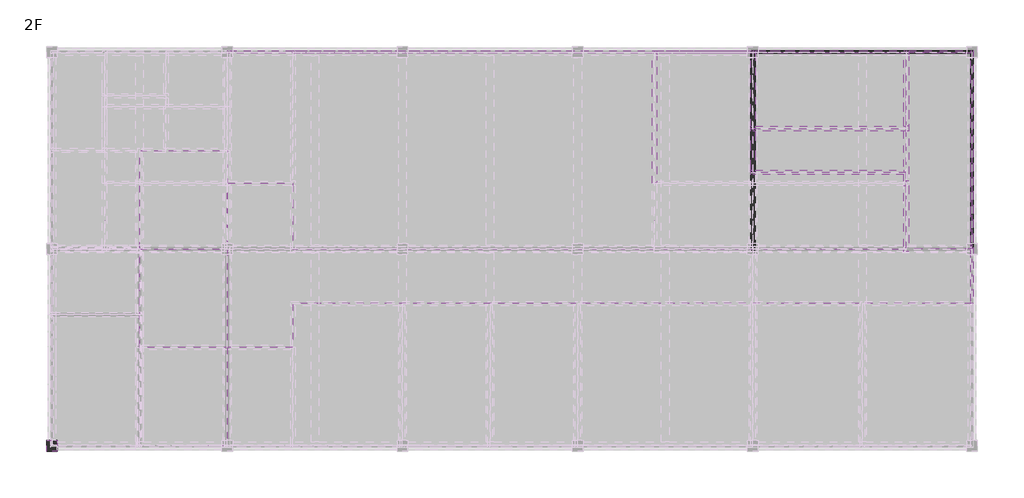
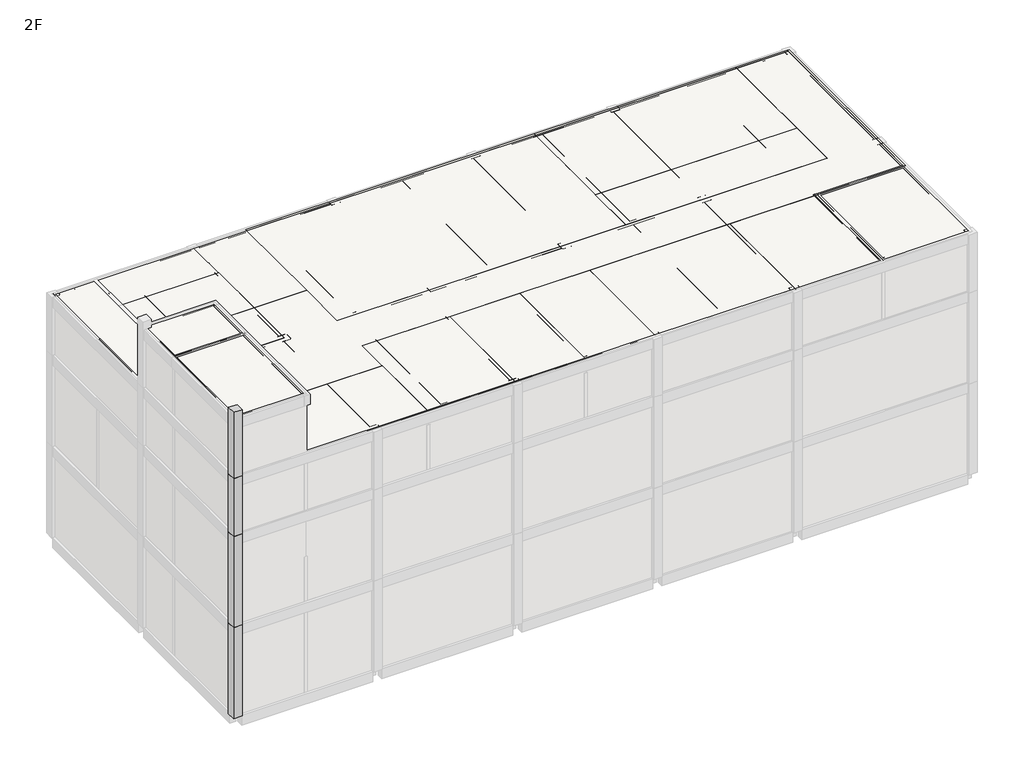
# One storey, part 3 of 7: 58 slabs, 19 walls, 4 columns.
"""IFC4 building model written with IfcOpenShell, lengths in millimetres."""

from ifc_helpers import new_model, si_unit, frame, origin, place, context, project, spatial, polyline, outline, extrude, faceted_brep, element, save

model = new_model("IFC4")

# Units and contexts
model_context = context("Model", 3, world=origin())
ifc_project = project(units=[si_unit("LENGTHUNIT", "METRE", prefix="MILLI")], contexts=[model_context])

# Site, building, storey
site = spatial("IfcSite", under=ifc_project)
building = spatial("IfcBuilding", under=site)
storey = spatial("IfcBuildingStorey", under=building, Name="2F", Elevation=3500.0)

# Columns
placement = place(None, origin())
element("IfcColumn", 1, ObjectType="Concrete-Rectangular-Column : CL111_500x500", at=placement, inside=storey, context=model_context, shape_type="Brep", body=[
    faceted_brep([(45709.6521483, 164173.8614395, 3500.0), (45709.6521483, 163673.8614395, 3500.0), (45209.6521483, 163673.8614395, 3500.0), (45209.6521483, 164173.8614395, 3500.0), (45709.6521483, 164173.8614395, 9000.0), (45709.6521483, 164098.8614395, 9000.0), (45709.6521483, 163748.8614395, 9000.0), (45709.6521483, 163673.8614395, 9000.0), (45209.6521483, 163673.8614395, 9000.0), (45209.6521483, 164173.8614395, 9000.0), (45284.6521483, 164173.8614395, 9000.0), (45634.6521483, 164173.8614395, 9000.0)], [[[0, 1, 2, 3]], [[4, 5, 6, 7, 1, 0]], [[7, 8, 2, 1]], [[8, 9, 3, 2]], [[9, 10, 11, 4, 0, 3]], [[4, 11, 10, 9, 8, 7, 6, 5]]]),
])
element("IfcColumn", 2, ObjectType="Concrete-Rectangular-Column : CL111_500x500", at=placement, inside=storey, context=model_context, shape_type="Brep", body=[
    faceted_brep([(45709.6521483, 164173.8614395, 9000.0), (45709.6521483, 163673.8614395, 9000.0), (45209.6521483, 163673.8614395, 9000.0), (45209.6521483, 164173.8614395, 9000.0), (45709.6521483, 164173.8614395, 14500.0), (45709.6521483, 164098.8614395, 14500.0), (45709.6521483, 163748.8614395, 14500.0), (45709.6521483, 163673.8614395, 14500.0), (45209.6521483, 163673.8614395, 14500.0), (45209.6521483, 164173.8614395, 14500.0), (45284.6521483, 164173.8614395, 14500.0), (45634.6521483, 164173.8614395, 14500.0)], [[[0, 1, 2, 3]], [[4, 5, 6, 7, 1, 0]], [[7, 8, 2, 1]], [[8, 9, 3, 2]], [[9, 10, 11, 4, 0, 3]], [[4, 11, 10, 9, 8, 7, 6, 5]]]),
])
element("IfcColumn", 3, ObjectType="Concrete-Rectangular-Column : CL111_500x500", at=placement, inside=storey, context=model_context, shape_type="Brep", body=[
    faceted_brep([(45709.6521483, 164173.8614395, 14500.0), (45709.6521483, 163673.8614395, 14500.0), (45209.6521483, 163673.8614395, 14500.0), (45209.6521483, 164173.8614395, 14500.0), (45709.6521483, 164173.8614395, 18000.0), (45709.6521483, 164098.8614395, 18000.0), (45709.6521483, 163748.8614395, 18000.0), (45709.6521483, 163673.8614395, 18000.0), (45209.6521483, 163673.8614395, 18000.0), (45209.6521483, 164173.8614395, 18000.0), (45284.6521483, 164173.8614395, 18000.0), (45634.6521483, 164173.8614395, 18000.0)], [[[0, 1, 2, 3]], [[4, 5, 6, 7, 1, 0]], [[7, 8, 2, 1]], [[8, 9, 3, 2]], [[9, 10, 11, 4, 0, 3]], [[4, 11, 10, 9, 8, 7, 6, 5]]]),
])
element("IfcColumn", 4, ObjectType="Concrete-Rectangular-Column : CL111_500x500", at=placement, inside=storey, context=model_context, shape_type="SweptSolid", body=[
    extrude(outline(polyline([(45709.6521483, 164173.8614395), (45709.6521483, 163673.8614395), (45209.6521483, 163673.8614395), (45209.6521483, 164173.8614395), (45709.6521483, 164173.8614395)])), frame((0.0, 0.0, 18000.0), z_axis=(0.0, 0.0, 1.0), x_axis=(1.0, 0.0, 0.0)), (0.0, 0.0, 1.0), 4000.0),
])

# Slabs
element("IfcSlab", 5, ObjectType="CFS11_Slab RC_T150", at=placement, inside=storey, context=model_context, shape_type="SweptSolid", body=[
    extrude(outline(polyline([(77459.6521483, 181923.8614395), (77459.6521483, 172923.8614395), (45459.6521483, 172923.8614395), (45459.6521483, 181923.8614395), (77459.6521483, 181923.8614395)])), frame((0.0, 0.0, 3350.0), z_axis=(0.0, 0.0, 1.0), x_axis=(1.0, 0.0, 0.0)), (0.0, 0.0, 1.0), 150.0),
])
element("IfcSlab", 6, ObjectType="CFS11_Slab RC_T150", at=placement, inside=storey, context=model_context, shape_type="SweptSolid", body=[
    extrude(outline(polyline([(53459.6521483, 163923.8614395), (53459.6521483, 172923.8614395), (87459.6521483, 172923.8614395), (87459.6521483, 163923.8614395), (53459.6521483, 163923.8614395)])), frame((0.0, 0.0, 3350.0), z_axis=(0.0, 0.0, 1.0), x_axis=(1.0, 0.0, 0.0)), (0.0, 0.0, 1.0), 150.0),
])
element("IfcSlab", 7, ObjectType="CFS11_Slab RC_T150", at=placement, inside=storey, context=model_context, shape_type="SweptSolid", body=[
    extrude(outline(polyline([(77459.6521483, 181923.8614395), (87459.6521483, 181923.8614395), (87459.6521483, 172923.8614395), (77459.6521483, 172923.8614395), (77459.6521483, 181923.8614395)])), frame((0.0, 0.0, 3350.0), z_axis=(0.0, 0.0, 1.0), x_axis=(1.0, 0.0, 0.0)), (0.0, 0.0, 1.0), 150.0),
])
element("IfcSlab", 8, ObjectType="CFS11_Slab RC_T150", at=placement, inside=storey, context=model_context, shape_type="SweptSolid", body=[
    extrude(outline(polyline([(53459.6521483, 172923.8614395), (53459.6521483, 163923.8614395), (49459.6521483, 163923.8614395), (49459.6521483, 172923.8614395), (53459.6521483, 172923.8614395)])), frame((0.0, 0.0, 3350.0), z_axis=(0.0, 0.0, 1.0), x_axis=(1.0, 0.0, 0.0)), (0.0, 0.0, 1.0), 150.0),
])
element("IfcSlab", 9, ObjectType="CFS11_Slab RC_T150", at=placement, inside=storey, context=model_context, shape_type="SweptSolid", body=[
    extrude(outline(polyline([(49459.6521483, 172923.8614395), (49459.6521483, 169923.8614395), (45459.6521483, 169923.8614395), (45459.6521483, 172923.8614395), (49459.6521483, 172923.8614395)])), frame((0.0, 0.0, 3350.0), z_axis=(0.0, 0.0, 1.0), x_axis=(1.0, 0.0, 0.0)), (0.0, 0.0, 1.0), 150.0),
])
element("IfcSlab", 10, ObjectType="CFS11_Slab RC_T150", at=placement, inside=storey, context=model_context, shape_type="SweptSolid", body=[
    extrude(outline(polyline([(49459.6521483, 163923.8614395), (45459.6521483, 163923.8614395), (45459.6521483, 169923.8614395), (49459.6521483, 169923.8614395), (49459.6521483, 163923.8614395)])), frame((0.0, 0.0, 3350.0), z_axis=(0.0, 0.0, 1.0), x_axis=(1.0, 0.0, 0.0)), (0.0, 0.0, 1.0), 150.0),
])
element("IfcSlab", 11, ObjectType="CFS11_Slab RC_T150", at=placement, inside=storey, context=model_context, shape_type="SweptSolid", body=[
    extrude(outline(polyline([(53459.6521483, 181923.8614395), (77459.6521483, 181923.8614395), (77459.6521483, 172923.8614395), (53459.6521483, 172923.8614395), (53459.6521483, 181923.8614395)])), frame((0.0, 0.0, 8850.0), z_axis=(0.0, 0.0, 1.0), x_axis=(1.0, 0.0, 0.0)), (0.0, 0.0, 1.0), 150.0),
])
element("IfcSlab", 12, ObjectType="CFS11_Slab RC_T150", at=placement, inside=storey, context=model_context, shape_type="SweptSolid", body=[
    extrude(outline(polyline([(77459.6521483, 172923.8614395), (77459.6521483, 163923.8614395), (53459.6521483, 163923.8614395), (53459.6521483, 172923.8614395), (77459.6521483, 172923.8614395)])), frame((0.0, 0.0, 8850.0), z_axis=(0.0, 0.0, 1.0), x_axis=(1.0, 0.0, 0.0)), (0.0, 0.0, 1.0), 150.0),
])
element("IfcSlab", 13, ObjectType="CFS11_Slab RC_T150", at=placement, inside=storey, context=model_context, shape_type="SweptSolid", body=[
    extrude(outline(polyline([(77459.6521483, 181923.8614395), (84459.6521483, 181923.8614395), (84459.6521483, 178423.8614395), (77459.6521483, 178423.8614395), (77459.6521483, 181923.8614395)])), frame((0.0, 0.0, 8850.0), z_axis=(0.0, 0.0, 1.0), x_axis=(1.0, 0.0, 0.0)), (0.0, 0.0, 1.0), 150.0),
])
element("IfcSlab", 14, ObjectType="CFS11_Slab RC_T150", at=placement, inside=storey, context=model_context, shape_type="SweptSolid", body=[
    extrude(outline(polyline([(77459.6521483, 163923.8614395), (77459.6521483, 172923.8614395), (87459.6521483, 172923.8614395), (87459.6521483, 163923.8614395), (77459.6521483, 163923.8614395)])), frame((0.0, 0.0, 8850.0), z_axis=(0.0, 0.0, 1.0), x_axis=(1.0, 0.0, 0.0)), (0.0, 0.0, 1.0), 150.0),
])
element("IfcSlab", 15, ObjectType="CFS11_Slab RC_T150", at=placement, inside=storey, context=model_context, shape_type="SweptSolid", body=[
    extrude(outline(polyline([(77459.6521483, 176423.8614395), (84459.6521483, 176423.8614395), (84459.6521483, 172923.8614395), (77459.6521483, 172923.8614395), (77459.6521483, 176423.8614395)])), frame((0.0, 0.0, 8850.0), z_axis=(0.0, 0.0, 1.0), x_axis=(1.0, 0.0, 0.0)), (0.0, 0.0, 1.0), 150.0),
])
element("IfcSlab", 16, ObjectType="CFS11_Slab RC_T150", at=placement, inside=storey, context=model_context, shape_type="SweptSolid", body=[
    extrude(outline(polyline([(45459.6521483, 181923.8614395), (47859.6521483, 181923.8614395), (47859.6521483, 177423.8614395), (45459.6521483, 177423.8614395), (45459.6521483, 181923.8614395)])), frame((0.0, 0.0, 8850.0), z_axis=(0.0, 0.0, 1.0), x_axis=(1.0, 0.0, 0.0)), (0.0, 0.0, 1.0), 150.0),
])
element("IfcSlab", 17, ObjectType="CFS11_Slab RC_T150", at=placement, inside=storey, context=model_context, shape_type="SweptSolid", body=[
    extrude(outline(polyline([(45459.6521483, 172923.8614395), (45459.6521483, 177423.8614395), (49459.6521483, 177423.8614395), (49459.6521483, 172923.8614395), (45459.6521483, 172923.8614395)])), frame((0.0, 0.0, 8850.0), z_axis=(0.0, 0.0, 1.0), x_axis=(1.0, 0.0, 0.0)), (0.0, 0.0, 1.0), 150.0),
])
element("IfcSlab", 18, ObjectType="CFS11_Slab RC_T150", at=placement, inside=storey, context=model_context, shape_type="SweptSolid", body=[
    extrude(outline(polyline([(53459.6521483, 177423.8614395), (50659.6521483, 177423.8614395), (50659.6521483, 181923.8614395), (53459.6521483, 181923.8614395), (53459.6521483, 177423.8614395)])), frame((0.0, 0.0, 8850.0), z_axis=(0.0, 0.0, 1.0), x_axis=(1.0, 0.0, 0.0)), (0.0, 0.0, 1.0), 150.0),
])
element("IfcSlab", 19, ObjectType="CFS11_Slab RC_T150", at=placement, inside=storey, context=model_context, shape_type="SweptSolid", body=[
    extrude(outline(polyline([(47859.6521483, 181923.8614395), (50659.6521483, 181923.8614395), (50659.6521483, 179923.8614395), (47859.6521483, 179923.8614395), (47859.6521483, 181923.8614395)])), frame((0.0, 0.0, 8850.0), z_axis=(0.0, 0.0, 1.0), x_axis=(1.0, 0.0, 0.0)), (0.0, 0.0, 1.0), 150.0),
])
element("IfcSlab", 20, ObjectType="CFS11_Slab RC_T150", at=placement, inside=storey, context=model_context, shape_type="SweptSolid", body=[
    extrude(outline(polyline([(47859.6521483, 179923.8614395), (50659.6521483, 179923.8614395), (50659.6521483, 177423.8614395), (47859.6521483, 177423.8614395), (47859.6521483, 179923.8614395)])), frame((0.0, 0.0, 8850.0), z_axis=(0.0, 0.0, 1.0), x_axis=(1.0, 0.0, 0.0)), (0.0, 0.0, 1.0), 150.0),
])
element("IfcSlab", 21, ObjectType="CFS11_Slab RC_T150", at=placement, inside=storey, context=model_context, shape_type="SweptSolid", body=[
    extrude(outline(polyline([(49459.6521483, 172923.8614395), (49459.6521483, 169923.8614395), (45459.6521483, 169923.8614395), (45459.6521483, 172923.8614395), (49459.6521483, 172923.8614395)])), frame((0.0, 0.0, 8850.0), z_axis=(0.0, 0.0, 1.0), x_axis=(1.0, 0.0, 0.0)), (0.0, 0.0, 1.0), 150.0),
])
element("IfcSlab", 22, ObjectType="CFS11_Slab RC_T150", at=placement, inside=storey, context=model_context, shape_type="SweptSolid", body=[
    extrude(outline(polyline([(49459.6521483, 169923.8614395), (49459.6521483, 163923.8614395), (45459.6521483, 163923.8614395), (45459.6521483, 169923.8614395), (49459.6521483, 169923.8614395)])), frame((0.0, 0.0, 8850.0), z_axis=(0.0, 0.0, 1.0), x_axis=(1.0, 0.0, 0.0)), (0.0, 0.0, 1.0), 150.0),
])
element("IfcSlab", 23, ObjectType="CFS11_Slab RC_T150", at=placement, inside=storey, context=model_context, shape_type="SweptSolid", body=[
    extrude(outline(polyline([(77459.6521483, 178423.8614395), (84459.6521483, 178423.8614395), (84459.6521483, 181923.8614395), (87459.6521483, 181923.8614395), (87459.6521483, 172923.8614395), (84459.6521483, 172923.8614395), (84459.6521483, 176423.8614395), (77459.6521483, 176423.8614395), (77459.6521483, 178423.8614395)])), frame((0.0, 0.0, 8850.0), z_axis=(0.0, 0.0, 1.0), x_axis=(1.0, 0.0, 0.0)), (0.0, 0.0, 1.0), 150.0),
])
element("IfcSlab", 24, ObjectType="CFS11_Slab RC_T150", at=placement, inside=storey, context=model_context, shape_type="SweptSolid", body=[
    extrude(outline(polyline([(49459.6521483, 177423.8614395), (53459.6521483, 177423.8614395), (53459.6521483, 163923.8614395), (49459.6521483, 163923.8614395), (49459.6521483, 177423.8614395)])), frame((0.0, 0.0, 8850.0), z_axis=(0.0, 0.0, 1.0), x_axis=(1.0, 0.0, 0.0)), (0.0, 0.0, 1.0), 150.0),
])
element("IfcSlab", 25, ObjectType="CFS11_Slab RC_T150", at=placement, inside=storey, context=model_context, shape_type="SweptSolid", body=[
    extrude(outline(polyline([(61459.6521483, 163923.8614395), (61459.6521483, 170423.8614395), (65459.6521483, 170423.8614395), (65459.6521483, 163923.8614395), (61459.6521483, 163923.8614395)])), frame((0.0, 0.0, 14350.0), z_axis=(0.0, 0.0, 1.0), x_axis=(1.0, 0.0, 0.0)), (0.0, 0.0, 1.0), 150.0),
])
element("IfcSlab", 26, ObjectType="CFS11_Slab RC_T150", at=placement, inside=storey, context=model_context, shape_type="SweptSolid", body=[
    extrude(outline(polyline([(65459.6521483, 170423.8614395), (69459.6521483, 170423.8614395), (69459.6521483, 163923.8614395), (65459.6521483, 163923.8614395), (65459.6521483, 170423.8614395)])), frame((0.0, 0.0, 14350.0), z_axis=(0.0, 0.0, 1.0), x_axis=(1.0, 0.0, 0.0)), (0.0, 0.0, 1.0), 150.0),
])
element("IfcSlab", 27, ObjectType="CFS11_Slab RC_T150", at=placement, inside=storey, context=model_context, shape_type="SweptSolid", body=[
    extrude(outline(polyline([(84459.6521483, 181923.8614395), (84459.6521483, 175923.8614395), (72959.6521483, 175923.8614395), (72959.6521483, 181923.8614395), (84459.6521483, 181923.8614395)])), frame((0.0, 0.0, 14350.0), z_axis=(0.0, 0.0, 1.0), x_axis=(1.0, 0.0, 0.0)), (0.0, 0.0, 1.0), 150.0),
])
element("IfcSlab", 28, ObjectType="CFS11_Slab RC_T150", at=placement, inside=storey, context=model_context, shape_type="SweptSolid", body=[
    extrude(outline(polyline([(69459.6521483, 170423.8614395), (77459.6521483, 170423.8614395), (77459.6521483, 163923.8614395), (69459.6521483, 163923.8614395), (69459.6521483, 170423.8614395)])), frame((0.0, 0.0, 14350.0), z_axis=(0.0, 0.0, 1.0), x_axis=(1.0, 0.0, 0.0)), (0.0, 0.0, 1.0), 150.0),
])
element("IfcSlab", 29, ObjectType="CFS11_Slab RC_T150", at=placement, inside=storey, context=model_context, shape_type="SweptSolid", body=[
    extrude(outline(polyline([(56459.6521483, 181923.8614395), (72959.6521483, 181923.8614395), (72959.6521483, 172923.8614395), (56459.6521483, 172923.8614395), (56459.6521483, 181923.8614395)])), frame((0.0, 0.0, 14350.0), z_axis=(0.0, 0.0, 1.0), x_axis=(1.0, 0.0, 0.0)), (0.0, 0.0, 1.0), 150.0),
])
element("IfcSlab", 30, ObjectType="CFS11_Slab RC_T150", at=placement, inside=storey, context=model_context, shape_type="SweptSolid", body=[
    extrude(outline(polyline([(77459.6521483, 170423.8614395), (82459.6521483, 170423.8614395), (82459.6521483, 163923.8614395), (77459.6521483, 163923.8614395), (77459.6521483, 170423.8614395)])), frame((0.0, 0.0, 14350.0), z_axis=(0.0, 0.0, 1.0), x_axis=(1.0, 0.0, 0.0)), (0.0, 0.0, 1.0), 150.0),
])
element("IfcSlab", 31, ObjectType="CFS11_Slab RC_T150", at=placement, inside=storey, context=model_context, shape_type="SweptSolid", body=[
    extrude(outline(polyline([(82459.6521483, 170423.8614395), (87459.6521483, 170423.8614395), (87459.6521483, 163923.8614395), (82459.6521483, 163923.8614395), (82459.6521483, 170423.8614395)])), frame((0.0, 0.0, 14350.0), z_axis=(0.0, 0.0, 1.0), x_axis=(1.0, 0.0, 0.0)), (0.0, 0.0, 1.0), 150.0),
])
element("IfcSlab", 32, ObjectType="CFS11_Slab RC_T150", at=placement, inside=storey, context=model_context, shape_type="SweptSolid", body=[
    extrude(outline(polyline([(84459.6521483, 175923.8614395), (84459.6521483, 172923.8614395), (72959.6521483, 172923.8614395), (72959.6521483, 175923.8614395), (84459.6521483, 175923.8614395)])), frame((0.0, 0.0, 14350.0), z_axis=(0.0, 0.0, 1.0), x_axis=(1.0, 0.0, 0.0)), (0.0, 0.0, 1.0), 150.0),
])
element("IfcSlab", 33, ObjectType="CFS11_Slab RC_T150", at=placement, inside=storey, context=model_context, shape_type="SweptSolid", body=[
    extrude(outline(polyline([(61459.6521483, 163923.8614395), (56459.6521483, 163923.8614395), (56459.6521483, 170423.8614395), (61459.6521483, 170423.8614395), (61459.6521483, 163923.8614395)])), frame((0.0, 0.0, 14350.0), z_axis=(0.0, 0.0, 1.0), x_axis=(1.0, 0.0, 0.0)), (0.0, 0.0, 1.0), 150.0),
])
element("IfcSlab", 34, ObjectType="CFS11_Slab RC_T150", at=placement, inside=storey, context=model_context, shape_type="SweptSolid", body=[
    extrude(outline(polyline([(56459.6521483, 163923.8614395), (49459.6521483, 163923.8614395), (49459.6521483, 168423.8614395), (56459.6521483, 168423.8614395), (56459.6521483, 163923.8614395)])), frame((0.0, 0.0, 14350.0), z_axis=(0.0, 0.0, 1.0), x_axis=(1.0, 0.0, 0.0)), (0.0, 0.0, 1.0), 150.0),
])
element("IfcSlab", 35, ObjectType="CFS11_Slab RC_T150", at=placement, inside=storey, context=model_context, shape_type="SweptSolid", body=[
    extrude(outline(polyline([(53459.6521483, 179423.8614395), (53459.6521483, 175923.8614395), (47859.6521483, 175923.8614395), (47859.6521483, 179423.8614395), (53459.6521483, 179423.8614395)])), frame((0.0, 0.0, 14350.0), z_axis=(0.0, 0.0, 1.0), x_axis=(1.0, 0.0, 0.0)), (0.0, 0.0, 1.0), 150.0),
])
element("IfcSlab", 36, ObjectType="CFS11_Slab RC_T150", at=placement, inside=storey, context=model_context, shape_type="SweptSolid", body=[
    extrude(outline(polyline([(47859.6521483, 179423.8614395), (47859.6521483, 181923.8614395), (53459.6521483, 181923.8614395), (53459.6521483, 179423.8614395), (47859.6521483, 179423.8614395)])), frame((0.0, 0.0, 14350.0), z_axis=(0.0, 0.0, 1.0), x_axis=(1.0, 0.0, 0.0)), (0.0, 0.0, 1.0), 150.0),
])
element("IfcSlab", 37, ObjectType="CFS11_Slab RC_T150", at=placement, inside=storey, context=model_context, shape_type="SweptSolid", body=[
    extrude(outline(polyline([(56459.6521483, 175923.8614395), (53459.6521483, 175923.8614395), (53459.6521483, 181923.8614395), (56459.6521483, 181923.8614395), (56459.6521483, 175923.8614395)])), frame((0.0, 0.0, 14350.0), z_axis=(0.0, 0.0, 1.0), x_axis=(1.0, 0.0, 0.0)), (0.0, 0.0, 1.0), 150.0),
])
element("IfcSlab", 38, ObjectType="CFS11_Slab RC_T150", at=placement, inside=storey, context=model_context, shape_type="SweptSolid", body=[
    extrude(outline(polyline([(53459.6521483, 175923.8614395), (53459.6521483, 172923.8614395), (47859.6521483, 172923.8614395), (47859.6521483, 175923.8614395), (53459.6521483, 175923.8614395)])), frame((0.0, 0.0, 14350.0), z_axis=(0.0, 0.0, 1.0), x_axis=(1.0, 0.0, 0.0)), (0.0, 0.0, 1.0), 150.0),
])
element("IfcSlab", 39, ObjectType="CFS11_Slab RC_T150", at=placement, inside=storey, context=model_context, shape_type="SweptSolid", body=[
    extrude(outline(polyline([(45459.6521483, 181923.8614395), (47859.6521483, 181923.8614395), (47859.6521483, 172923.8614395), (45459.6521483, 172923.8614395), (45459.6521483, 181923.8614395)])), frame((0.0, 0.0, 14350.0), z_axis=(0.0, 0.0, 1.0), x_axis=(1.0, 0.0, 0.0)), (0.0, 0.0, 1.0), 150.0),
])
element("IfcSlab", 40, ObjectType="CFS11_Slab RC_T150", at=placement, inside=storey, context=model_context, shape_type="SweptSolid", body=[
    extrude(outline(polyline([(49459.6521483, 172923.8614395), (49459.6521483, 169923.8614395), (45459.6521483, 169923.8614395), (45459.6521483, 172923.8614395), (49459.6521483, 172923.8614395)])), frame((0.0, 0.0, 14350.0), z_axis=(0.0, 0.0, 1.0), x_axis=(1.0, 0.0, 0.0)), (0.0, 0.0, 1.0), 150.0),
])
element("IfcSlab", 41, ObjectType="CFS11_Slab RC_T150", at=placement, inside=storey, context=model_context, shape_type="SweptSolid", body=[
    extrude(outline(polyline([(49459.6521483, 163923.8614395), (45459.6521483, 163923.8614395), (45459.6521483, 169923.8614395), (49459.6521483, 169923.8614395), (49459.6521483, 163923.8614395)])), frame((0.0, 0.0, 14350.0), z_axis=(0.0, 0.0, 1.0), x_axis=(1.0, 0.0, 0.0)), (0.0, 0.0, 1.0), 150.0),
])
element("IfcSlab", 42, ObjectType="CFS11_Slab RC_T150", at=placement, inside=storey, context=model_context, shape_type="SweptSolid", body=[
    extrude(outline(polyline([(87459.6521483, 181923.8614395), (87459.6521483, 170423.8614395), (56459.6521483, 170423.8614395), (56459.6521483, 168423.8614395), (49459.6521483, 168423.8614395), (49459.6521483, 172923.8614395), (53459.6521483, 172923.8614395), (53459.6521483, 175923.8614395), (56459.6521483, 175923.8614395), (56459.6521483, 172923.8614395), (84459.6521483, 172923.8614395), (84459.6521483, 181923.8614395), (87459.6521483, 181923.8614395)])), frame((0.0, 0.0, 14350.0), z_axis=(0.0, 0.0, 1.0), x_axis=(1.0, 0.0, 0.0)), (0.0, 0.0, 1.0), 150.0),
])
element("IfcSlab", 43, ObjectType="CFS11_Slab RC_T150", at=placement, inside=storey, context=model_context, shape_type="SweptSolid", body=[
    extrude(outline(polyline([(45459.6521483, 172923.8614395), (49459.6521483, 172923.8614395), (49459.6521483, 169923.8614395), (45459.6521483, 169923.8614395), (45459.6521483, 172923.8614395)])), frame((0.0, 0.0, 17850.0), z_axis=(0.0, 0.0, 1.0), x_axis=(1.0, 0.0, 0.0)), (0.0, 0.0, 1.0), 150.0),
])
element("IfcSlab", 44, ObjectType="CFS11_Slab RC_T150", at=placement, inside=storey, context=model_context, shape_type="SweptSolid", body=[
    extrude(outline(polyline([(49459.6521483, 169923.8614395), (49459.6521483, 163923.8614395), (45459.6521483, 163923.8614395), (45459.6521483, 169923.8614395), (49459.6521483, 169923.8614395)])), frame((0.0, 0.0, 17850.0), z_axis=(0.0, 0.0, 1.0), x_axis=(1.0, 0.0, 0.0)), (0.0, 0.0, 1.0), 150.0),
])
element("IfcSlab", 45, ObjectType="CFS11_Slab RC_T150", at=placement, inside=storey, context=model_context, shape_type="SweptSolid", body=[
    extrude(outline(polyline([(61459.6521483, 163923.8614395), (61459.6521483, 170423.8614395), (65459.6521483, 170423.8614395), (65459.6521483, 163923.8614395), (61459.6521483, 163923.8614395)])), frame((0.0, 0.0, 17850.0), z_axis=(0.0, 0.0, 1.0), x_axis=(1.0, 0.0, 0.0)), (0.0, 0.0, 1.0), 150.0),
])
element("IfcSlab", 46, ObjectType="CFS11_Slab RC_T150", at=placement, inside=storey, context=model_context, shape_type="SweptSolid", body=[
    extrude(outline(polyline([(65459.6521483, 170423.8614395), (69459.6521483, 170423.8614395), (69459.6521483, 163923.8614395), (65459.6521483, 163923.8614395), (65459.6521483, 170423.8614395)])), frame((0.0, 0.0, 17850.0), z_axis=(0.0, 0.0, 1.0), x_axis=(1.0, 0.0, 0.0)), (0.0, 0.0, 1.0), 150.0),
])
element("IfcSlab", 47, ObjectType="CFS11_Slab RC_T150", at=placement, inside=storey, context=model_context, shape_type="SweptSolid", body=[
    extrude(outline(polyline([(84459.6521483, 181923.8614395), (84459.6521483, 175923.8614395), (72959.6521483, 175923.8614395), (72959.6521483, 181923.8614395), (84459.6521483, 181923.8614395)])), frame((0.0, 0.0, 17850.0), z_axis=(0.0, 0.0, 1.0), x_axis=(1.0, 0.0, 0.0)), (0.0, 0.0, 1.0), 150.0),
])
element("IfcSlab", 48, ObjectType="CFS11_Slab RC_T150", at=placement, inside=storey, context=model_context, shape_type="SweptSolid", body=[
    extrude(outline(polyline([(69459.6521483, 170423.8614395), (77459.6521483, 170423.8614395), (77459.6521483, 163923.8614395), (69459.6521483, 163923.8614395), (69459.6521483, 170423.8614395)])), frame((0.0, 0.0, 17850.0), z_axis=(0.0, 0.0, 1.0), x_axis=(1.0, 0.0, 0.0)), (0.0, 0.0, 1.0), 150.0),
])
element("IfcSlab", 49, ObjectType="CFS11_Slab RC_T150", at=placement, inside=storey, context=model_context, shape_type="SweptSolid", body=[
    extrude(outline(polyline([(56459.6521483, 181923.8614395), (72959.6521483, 181923.8614395), (72959.6521483, 172923.8614395), (56459.6521483, 172923.8614395), (56459.6521483, 181923.8614395)])), frame((0.0, 0.0, 17850.0), z_axis=(0.0, 0.0, 1.0), x_axis=(1.0, 0.0, 0.0)), (0.0, 0.0, 1.0), 150.0),
])
element("IfcSlab", 50, ObjectType="CFS11_Slab RC_T150", at=placement, inside=storey, context=model_context, shape_type="SweptSolid", body=[
    extrude(outline(polyline([(77459.6521483, 170423.8614395), (82459.6521483, 170423.8614395), (82459.6521483, 163923.8614395), (77459.6521483, 163923.8614395), (77459.6521483, 170423.8614395)])), frame((0.0, 0.0, 17850.0), z_axis=(0.0, 0.0, 1.0), x_axis=(1.0, 0.0, 0.0)), (0.0, 0.0, 1.0), 150.0),
])
element("IfcSlab", 51, ObjectType="CFS11_Slab RC_T150", at=placement, inside=storey, context=model_context, shape_type="SweptSolid", body=[
    extrude(outline(polyline([(82459.6521483, 170423.8614395), (87459.6521483, 170423.8614395), (87459.6521483, 163923.8614395), (82459.6521483, 163923.8614395), (82459.6521483, 170423.8614395)])), frame((0.0, 0.0, 17850.0), z_axis=(0.0, 0.0, 1.0), x_axis=(1.0, 0.0, 0.0)), (0.0, 0.0, 1.0), 150.0),
])
element("IfcSlab", 52, ObjectType="CFS11_Slab RC_T150", at=placement, inside=storey, context=model_context, shape_type="SweptSolid", body=[
    extrude(outline(polyline([(84459.6521483, 175923.8614395), (84459.6521483, 172923.8614395), (72959.6521483, 172923.8614395), (72959.6521483, 175923.8614395), (84459.6521483, 175923.8614395)])), frame((0.0, 0.0, 17850.0), z_axis=(0.0, 0.0, 1.0), x_axis=(1.0, 0.0, 0.0)), (0.0, 0.0, 1.0), 150.0),
])
element("IfcSlab", 53, ObjectType="CFS11_Slab RC_T150", at=placement, inside=storey, context=model_context, shape_type="SweptSolid", body=[
    extrude(outline(polyline([(61459.6521483, 163923.8614395), (56459.6521483, 163923.8614395), (56459.6521483, 170423.8614395), (61459.6521483, 170423.8614395), (61459.6521483, 163923.8614395)])), frame((0.0, 0.0, 17850.0), z_axis=(0.0, 0.0, 1.0), x_axis=(1.0, 0.0, 0.0)), (0.0, 0.0, 1.0), 150.0),
])
element("IfcSlab", 54, ObjectType="CFS11_Slab RC_T150", at=placement, inside=storey, context=model_context, shape_type="SweptSolid", body=[
    extrude(outline(polyline([(56459.6521483, 163923.8614395), (49459.6521483, 163923.8614395), (49459.6521483, 168423.8614395), (56459.6521483, 168423.8614395), (56459.6521483, 163923.8614395)])), frame((0.0, 0.0, 17850.0), z_axis=(0.0, 0.0, 1.0), x_axis=(1.0, 0.0, 0.0)), (0.0, 0.0, 1.0), 150.0),
])
element("IfcSlab", 55, ObjectType="CFS11_Slab RC_T150", at=placement, inside=storey, context=model_context, shape_type="SweptSolid", body=[
    extrude(outline(polyline([(53459.6521483, 179423.8614395), (53459.6521483, 175923.8614395), (47859.6521483, 175923.8614395), (47859.6521483, 179423.8614395), (53459.6521483, 179423.8614395)])), frame((0.0, 0.0, 17850.0), z_axis=(0.0, 0.0, 1.0), x_axis=(1.0, 0.0, 0.0)), (0.0, 0.0, 1.0), 150.0),
])
element("IfcSlab", 56, ObjectType="CFS11_Slab RC_T150", at=placement, inside=storey, context=model_context, shape_type="SweptSolid", body=[
    extrude(outline(polyline([(47859.6521483, 179423.8614395), (47859.6521483, 181923.8614395), (53459.6521483, 181923.8614395), (53459.6521483, 179423.8614395), (47859.6521483, 179423.8614395)])), frame((0.0, 0.0, 17850.0), z_axis=(0.0, 0.0, 1.0), x_axis=(1.0, 0.0, 0.0)), (0.0, 0.0, 1.0), 150.0),
])
element("IfcSlab", 57, ObjectType="CFS11_Slab RC_T150", at=placement, inside=storey, context=model_context, shape_type="SweptSolid", body=[
    extrude(outline(polyline([(56459.6521483, 175923.8614395), (53459.6521483, 175923.8614395), (53459.6521483, 181923.8614395), (56459.6521483, 181923.8614395), (56459.6521483, 175923.8614395)])), frame((0.0, 0.0, 17850.0), z_axis=(0.0, 0.0, 1.0), x_axis=(1.0, 0.0, 0.0)), (0.0, 0.0, 1.0), 150.0),
])
element("IfcSlab", 58, ObjectType="CFS11_Slab RC_T150", at=placement, inside=storey, context=model_context, shape_type="SweptSolid", body=[
    extrude(outline(polyline([(53459.6521483, 175923.8614395), (53459.6521483, 172923.8614395), (47859.6521483, 172923.8614395), (47859.6521483, 175923.8614395), (53459.6521483, 175923.8614395)])), frame((0.0, 0.0, 17850.0), z_axis=(0.0, 0.0, 1.0), x_axis=(1.0, 0.0, 0.0)), (0.0, 0.0, 1.0), 150.0),
])
element("IfcSlab", 59, ObjectType="CFS11_Slab RC_T150", at=placement, inside=storey, context=model_context, shape_type="SweptSolid", body=[
    extrude(outline(polyline([(45459.6521483, 181923.8614395), (47859.6521483, 181923.8614395), (47859.6521483, 172923.8614395), (45459.6521483, 172923.8614395), (45459.6521483, 181923.8614395)])), frame((0.0, 0.0, 17850.0), z_axis=(0.0, 0.0, 1.0), x_axis=(1.0, 0.0, 0.0)), (0.0, 0.0, 1.0), 150.0),
])
element("IfcSlab", 60, ObjectType="CFS11_Slab RC_T150", at=placement, inside=storey, context=model_context, shape_type="SweptSolid", body=[
    extrude(outline(polyline([(87459.6521483, 181923.8614395), (87459.6521483, 170423.8614395), (56459.6521483, 170423.8614395), (56459.6521483, 168423.8614395), (49459.6521483, 168423.8614395), (49459.6521483, 172923.8614395), (53459.6521483, 172923.8614395), (53459.6521483, 175923.8614395), (56459.6521483, 175923.8614395), (56459.6521483, 172923.8614395), (84459.6521483, 172923.8614395), (84459.6521483, 181923.8614395), (87459.6521483, 181923.8614395)])), frame((0.0, 0.0, 17850.0), z_axis=(0.0, 0.0, 1.0), x_axis=(1.0, 0.0, 0.0)), (0.0, 0.0, 1.0), 150.0),
])
element("IfcSlab", 61, ObjectType="CFS11_Slab RC_T150", at=placement, inside=storey, context=model_context, shape_type="SweptSolid", body=[
    extrude(outline(polyline([(45459.6521483, 172923.8614395), (49459.6521483, 172923.8614395), (49459.6521483, 169923.8614395), (45459.6521483, 169923.8614395), (45459.6521483, 172923.8614395)])), frame((0.0, 0.0, 21350.0), z_axis=(0.0, 0.0, 1.0), x_axis=(1.0, 0.0, 0.0)), (0.0, 0.0, 1.0), 150.0),
])
element("IfcSlab", 62, ObjectType="CFS11_Slab RC_T150", at=placement, inside=storey, context=model_context, shape_type="SweptSolid", body=[
    extrude(outline(polyline([(49459.6521483, 169923.8614395), (49459.6521483, 163923.8614395), (45459.6521483, 163923.8614395), (45459.6521483, 169923.8614395), (49459.6521483, 169923.8614395)])), frame((0.0, 0.0, 21350.0), z_axis=(0.0, 0.0, 1.0), x_axis=(1.0, 0.0, 0.0)), (0.0, 0.0, 1.0), 150.0),
])

# Walls
element("IfcWall", 63, ObjectType="WA211_Exterior-Cement Brick-90mm", at=placement, inside=storey, context=model_context, shape_type="Brep", body=[
    faceted_brep([(87402.6521483, 181980.8614395, 3500.0), (87402.6521483, 181866.8614395, 3500.0), (87402.6521483, 173030.8614395, 3500.0), (87402.6521483, 172923.8614395, 3500.0), (87402.6521483, 172923.8614395, 9000.0), (87402.6521483, 173030.8614395, 9000.0), (87402.6521483, 181866.8614395, 9000.0), (87402.6521483, 181980.8614395, 9000.0), (87516.6521483, 181980.8614395, 3500.0), (87516.6521483, 181980.8614395, 9000.0), (87516.6521483, 172923.8614395, 9000.0), (87516.6521483, 172923.8614395, 3500.0)], [[[0, 1, 2, 3, 4, 5, 6, 7]], [[8, 9, 10, 11]], [[3, 2, 1, 0, 8, 11]], [[4, 3, 11, 10]], [[7, 6, 5, 4, 10, 9]], [[0, 7, 9, 8]]]),
])
element("IfcWall", 64, ObjectType="WA211_Exterior-Cement Brick-90mm", at=placement, inside=storey, context=model_context, shape_type="SweptSolid", body=[
    extrude(outline(polyline([(87402.6521483, 181866.8614395), (77566.6521483, 181866.8614395), (77566.6521483, 181980.8614395), (87402.6521483, 181980.8614395), (87402.6521483, 181866.8614395)])), frame((0.0, 0.0, 3500.0), z_axis=(0.0, 0.0, 1.0), x_axis=(1.0, 0.0, 0.0)), (0.0, 0.0, 1.0), 5500.0),
])
element("IfcWall", 65, ObjectType="WA211_Exterior-Cement Brick-90mm", at=placement, inside=storey, context=model_context, shape_type="SweptSolid", body=[
    extrude(outline(polyline([(9000.0, 53566.6521483), (9000.0, 77352.6521483), (12400.0, 77352.6521483), (12400.0, 77459.6521483), (14500.0, 77459.6521483), (14500.0, 53459.6521483), (12400.0, 53459.6521483), (12400.0, 53566.6521483), (9000.0, 53566.6521483)])), frame((0.0, 181866.8614395, 0.0), z_axis=(0.0, 1.0, 0.0), x_axis=(0.0, 0.0, 1.0)), (0.0, 0.0, 1.0), 114.0),
])
element("IfcWall", 66, ObjectType="WA211_Exterior-Cement Brick-90mm", at=placement, inside=storey, context=model_context, shape_type="SweptSolid", body=[
    extrude(outline(polyline([(9000.0, 77566.6521483), (9000.0, 84352.6521483), (11700.0, 84352.6521483), (11700.0, 84459.6521483), (14500.0, 84459.6521483), (14500.0, 77459.6521483), (12400.0, 77459.6521483), (12400.0, 77566.6521483), (9000.0, 77566.6521483)])), frame((0.0, 181866.8614395, 0.0), z_axis=(0.0, 1.0, 0.0), x_axis=(0.0, 0.0, 1.0)), (0.0, 0.0, 1.0), 114.0),
])
element("IfcWall", 67, ObjectType="WA211_Exterior-Cement Brick-90mm", at=placement, inside=storey, context=model_context, shape_type="Brep", body=[
    faceted_brep([(87402.6521483, 181980.8614395, 9000.0), (87402.6521483, 181866.8614395, 9000.0), (87402.6521483, 173030.8614395, 9000.0), (87402.6521483, 172923.8614395, 9000.0), (87402.6521483, 172923.8614395, 14500.0), (87402.6521483, 173030.8614395, 14500.0), (87402.6521483, 181866.8614395, 14500.0), (87402.6521483, 181980.8614395, 14500.0), (87516.6521483, 181980.8614395, 9000.0), (87516.6521483, 181980.8614395, 14500.0), (87516.6521483, 172923.8614395, 14500.0), (87516.6521483, 172923.8614395, 9000.0)], [[[0, 1, 2, 3, 4, 5, 6, 7]], [[8, 9, 10, 11]], [[3, 2, 1, 0, 8, 11]], [[4, 3, 11, 10]], [[7, 6, 5, 4, 10, 9]], [[0, 7, 9, 8]]]),
])
element("IfcWall", 68, ObjectType="WA211_Exterior-Cement Brick-90mm", at=placement, inside=storey, context=model_context, shape_type="SweptSolid", body=[
    extrude(outline(polyline([(9000.0, 84566.6521483), (9000.0, 87402.6521483), (14500.0, 87402.6521483), (14500.0, 84459.6521483), (11700.0, 84459.6521483), (11700.0, 84566.6521483), (9000.0, 84566.6521483)])), frame((0.0, 181866.8614395, 0.0), z_axis=(0.0, 1.0, 0.0), x_axis=(0.0, 0.0, 1.0)), (0.0, 0.0, 1.0), 114.0),
])
element("IfcWall", 69, ObjectType="WA211_Exterior-Cement Brick-90mm", at=placement, inside=storey, context=model_context, shape_type="SweptSolid", body=[
    extrude(outline(polyline([(14500.0, 73066.6521483), (14500.0, 84352.6521483), (17200.0, 84352.6521483), (17200.0, 84459.6521483), (18000.0, 84459.6521483), (18000.0, 72959.6521483), (17200.0, 72959.6521483), (17200.0, 73066.6521483), (14500.0, 73066.6521483)])), frame((0.0, 181866.8614395, 0.0), z_axis=(0.0, 1.0, 0.0), x_axis=(0.0, 0.0, 1.0)), (0.0, 0.0, 1.0), 114.0),
])
element("IfcWall", 70, ObjectType="WA211_Exterior-Cement Brick-90mm", at=placement, inside=storey, context=model_context, shape_type="SweptSolid", body=[
    extrude(outline(polyline([(14500.0, 56566.6521483), (14500.0, 72852.6521483), (17200.0, 72852.6521483), (17200.0, 72959.6521483), (18000.0, 72959.6521483), (18000.0, 56459.6521483), (17200.0, 56459.6521483), (17200.0, 56566.6521483), (14500.0, 56566.6521483)])), frame((0.0, 181866.8614395, 0.0), z_axis=(0.0, 1.0, 0.0), x_axis=(0.0, 0.0, 1.0)), (0.0, 0.0, 1.0), 114.0),
])
element("IfcWall", 71, ObjectType="WA211_Exterior-Cement Brick-90mm", at=placement, inside=storey, context=model_context, shape_type="Brep", body=[
    faceted_brep([(87402.6521483, 181980.8614395, 14500.0), (87402.6521483, 181866.8614395, 14500.0), (87402.6521483, 170530.8614395, 14500.0), (87402.6521483, 170423.8614395, 14500.0), (87402.6521483, 170423.8614395, 18000.0), (87402.6521483, 170530.8614395, 18000.0), (87402.6521483, 181866.8614395, 18000.0), (87402.6521483, 181980.8614395, 18000.0), (87516.6521483, 181980.8614395, 14500.0), (87516.6521483, 181980.8614395, 18000.0), (87516.6521483, 170423.8614395, 18000.0), (87516.6521483, 170423.8614395, 14500.0)], [[[0, 1, 2, 3, 4, 5, 6, 7]], [[8, 9, 10, 11]], [[3, 2, 1, 0, 8, 11]], [[4, 3, 11, 10]], [[7, 6, 5, 4, 10, 9]], [[0, 7, 9, 8]]]),
])
element("IfcWall", 72, ObjectType="WA211_Exterior-Cement Brick-90mm", at=placement, inside=storey, context=model_context, shape_type="SweptSolid", body=[
    extrude(outline(polyline([(14500.0, 84566.6521483), (14500.0, 87402.6521483), (18000.0, 87402.6521483), (18000.0, 84459.6521483), (17200.0, 84459.6521483), (17200.0, 84566.6521483), (14500.0, 84566.6521483)])), frame((0.0, 181866.8614395, 0.0), z_axis=(0.0, 1.0, 0.0), x_axis=(0.0, 0.0, 1.0)), (0.0, 0.0, 1.0), 114.0),
])
element("IfcWall", 73, ObjectType="WA221_Interior-Cement Block-190mm", at=placement, inside=storey, context=model_context, shape_type="Brep", body=[
    faceted_brep([(77566.6521483, 172816.8614395, 3500.0), (77566.6521483, 173030.8614395, 3500.0), (77566.6521483, 181866.8614395, 3500.0), (77566.6521483, 181980.8614395, 3500.0), (77566.6521483, 181980.8614395, 9000.0), (77566.6521483, 181866.8614395, 9000.0), (77566.6521483, 173030.8614395, 9000.0), (77566.6521483, 172816.8614395, 9000.0), (77352.6521483, 172816.8614395, 3500.0), (77352.6521483, 172816.8614395, 9000.0), (77352.6521483, 173030.8614395, 9000.0), (77352.6521483, 181866.8614395, 9000.0), (77352.6521483, 181980.8614395, 9000.0), (77352.6521483, 181980.8614395, 3500.0), (77352.6521483, 181866.8614395, 3500.0), (77352.6521483, 173030.8614395, 3500.0)], [[[0, 1, 2, 3, 4, 5, 6, 7]], [[8, 9, 10, 11, 12, 13, 14, 15]], [[3, 2, 1, 0, 8, 15, 14, 13]], [[7, 6, 5, 4, 12, 11, 10, 9]], [[0, 7, 9, 8]], [[4, 3, 13, 12]]]),
])
element("IfcWall", 74, ObjectType="WA221_Interior-Cement Block-190mm", at=placement, inside=storey, context=model_context, shape_type="Brep", body=[
    faceted_brep([(77352.6521483, 181980.8614395, 9000.0), (77352.6521483, 181866.8614395, 9000.0), (77352.6521483, 178530.8614395, 9000.0), (77352.6521483, 178530.8614395, 11700.0), (77352.6521483, 178423.8614395, 11700.0), (77352.6521483, 178423.8614395, 12400.0), (77352.6521483, 181866.8614395, 12400.0), (77352.6521483, 181980.8614395, 12400.0), (77566.6521483, 181980.8614395, 9000.0), (77566.6521483, 181980.8614395, 12400.0), (77566.6521483, 181866.8614395, 12400.0), (77566.6521483, 178423.8614395, 12400.0), (77566.6521483, 178423.8614395, 11700.0), (77566.6521483, 178530.8614395, 11700.0), (77566.6521483, 178530.8614395, 9000.0), (77566.6521483, 181866.8614395, 9000.0), (77459.6521483, 181980.8614395, 12400.0)], [[[0, 1, 2, 3, 4, 5, 6, 7]], [[8, 9, 10, 11, 12, 13, 14, 15]], [[2, 1, 0, 8, 15, 14]], [[7, 6, 5, 11, 10, 9, 16]], [[0, 7, 16, 9, 8]], [[5, 4, 12, 11]], [[12, 4, 3, 13]], [[3, 2, 14, 13]]]),
])
element("IfcWall", 75, ObjectType="WA221_Interior-Cement Block-190mm", at=placement, inside=storey, context=model_context, shape_type="SweptSolid", body=[
    extrude(outline(polyline([(178316.8614395, 9000.0), (176530.8614395, 9000.0), (176530.8614395, 11700.0), (176423.8614395, 11700.0), (176423.8614395, 12400.0), (178423.8614395, 12400.0), (178423.8614395, 11700.0), (178316.8614395, 11700.0), (178316.8614395, 9000.0)])), frame((77352.6521483, 0.0, 0.0), z_axis=(1.0, 0.0, 0.0), x_axis=(0.0, 1.0, 0.0)), (0.0, 0.0, 1.0), 214.0),
])
element("IfcWall", 76, ObjectType="WA221_Interior-Cement Block-190mm", at=placement, inside=storey, context=model_context, shape_type="Brep", body=[
    faceted_brep([(84566.6521483, 178530.8614395, 9000.0), (84352.6521483, 178530.8614395, 9000.0), (77566.6521483, 178530.8614395, 9000.0), (77352.6521483, 178530.8614395, 9000.0), (77352.6521483, 178530.8614395, 11700.0), (77566.6521483, 178530.8614395, 11700.0), (84352.6521483, 178530.8614395, 11700.0), (84566.6521483, 178530.8614395, 11700.0), (84566.6521483, 178316.8614395, 9000.0), (84566.6521483, 178316.8614395, 11700.0), (77566.6521483, 178316.8614395, 11700.0), (77352.6521483, 178316.8614395, 11700.0), (77352.6521483, 178316.8614395, 9000.0), (77566.6521483, 178316.8614395, 9000.0), (77352.6521483, 178423.8614395, 11700.0)], [[[0, 1, 2, 3, 4, 5, 6, 7]], [[8, 9, 10, 11, 12, 13]], [[3, 2, 1, 0, 8, 13, 12]], [[7, 6, 5, 4, 14, 11, 10, 9]], [[0, 7, 9, 8]], [[4, 3, 12, 11, 14]]]),
])
element("IfcWall", 77, ObjectType="WA221_Interior-Cement Block-190mm", at=placement, inside=storey, context=model_context, shape_type="Brep", body=[
    faceted_brep([(84352.6521483, 181980.8614395, 9000.0), (84352.6521483, 181866.8614395, 9000.0), (84352.6521483, 178530.8614395, 9000.0), (84352.6521483, 178530.8614395, 11700.0), (84352.6521483, 181866.8614395, 11700.0), (84352.6521483, 181980.8614395, 11700.0), (84566.6521483, 181980.8614395, 9000.0), (84566.6521483, 181980.8614395, 11700.0), (84566.6521483, 181866.8614395, 11700.0), (84566.6521483, 178530.8614395, 11700.0), (84566.6521483, 178530.8614395, 9000.0), (84566.6521483, 181866.8614395, 9000.0), (84459.6521483, 181980.8614395, 11700.0)], [[[0, 1, 2, 3, 4, 5]], [[6, 7, 8, 9, 10, 11]], [[2, 1, 0, 6, 11, 10]], [[5, 4, 3, 9, 8, 7, 12]], [[0, 5, 12, 7, 6]], [[3, 2, 10, 9]]]),
])
element("IfcWall", 78, ObjectType="WA221_Interior-Cement Block-190mm", at=placement, inside=storey, context=model_context, shape_type="Brep", body=[
    faceted_brep([(84352.6521483, 176530.8614395, 9000.0), (77566.6521483, 176530.8614395, 9000.0), (77352.6521483, 176530.8614395, 9000.0), (77352.6521483, 176530.8614395, 11700.0), (77566.6521483, 176530.8614395, 11700.0), (84352.6521483, 176530.8614395, 11700.0), (84352.6521483, 176316.8614395, 9000.0), (84352.6521483, 176316.8614395, 11700.0), (77566.6521483, 176316.8614395, 11700.0), (77352.6521483, 176316.8614395, 11700.0), (77352.6521483, 176316.8614395, 9000.0), (77566.6521483, 176316.8614395, 9000.0), (77352.6521483, 176423.8614395, 11700.0)], [[[0, 1, 2, 3, 4, 5]], [[6, 7, 8, 9, 10, 11]], [[2, 1, 0, 6, 11, 10]], [[5, 4, 3, 12, 9, 8, 7]], [[3, 2, 10, 9, 12]], [[0, 5, 7, 6]]]),
])
element("IfcWall", 79, ObjectType="WA221_Interior-Cement Block-190mm", at=placement, inside=storey, context=model_context, shape_type="Brep", body=[
    faceted_brep([(73066.6521483, 175923.8614395, 14500.0), (73066.6521483, 176030.8614395, 14500.0), (73066.6521483, 181866.8614395, 14500.0), (73066.6521483, 181980.8614395, 14500.0), (73066.6521483, 181980.8614395, 17200.0), (73066.6521483, 181866.8614395, 17200.0), (73066.6521483, 176030.8614395, 17200.0), (73066.6521483, 175923.8614395, 17200.0), (72852.6521483, 175923.8614395, 14500.0), (72852.6521483, 175923.8614395, 17200.0), (72852.6521483, 181866.8614395, 17200.0), (72852.6521483, 181980.8614395, 17200.0), (72852.6521483, 181980.8614395, 14500.0), (72852.6521483, 181866.8614395, 14500.0), (72959.6521483, 181980.8614395, 17200.0)], [[[0, 1, 2, 3, 4, 5, 6, 7]], [[8, 9, 10, 11, 12, 13]], [[3, 2, 1, 0, 8, 13, 12]], [[7, 6, 5, 4, 14, 11, 10, 9]], [[0, 7, 9, 8]], [[4, 3, 12, 11, 14]]]),
])
element("IfcWall", 80, ObjectType="WA221_Interior-Cement Block-190mm", at=placement, inside=storey, context=model_context, shape_type="Brep", body=[
    faceted_brep([(84352.6521483, 181980.8614395, 14500.0), (84352.6521483, 181866.8614395, 14500.0), (84352.6521483, 176030.8614395, 14500.0), (84352.6521483, 176030.8614395, 17200.0), (84352.6521483, 181866.8614395, 17200.0), (84352.6521483, 181980.8614395, 17200.0), (84566.6521483, 181980.8614395, 14500.0), (84566.6521483, 181980.8614395, 17200.0), (84566.6521483, 181866.8614395, 17200.0), (84566.6521483, 176030.8614395, 17200.0), (84566.6521483, 176030.8614395, 14500.0), (84566.6521483, 181866.8614395, 14500.0), (84459.6521483, 181980.8614395, 17200.0)], [[[0, 1, 2, 3, 4, 5]], [[6, 7, 8, 9, 10, 11]], [[2, 1, 0, 6, 11, 10]], [[5, 4, 3, 9, 8, 7, 12]], [[0, 5, 12, 7, 6]], [[3, 2, 10, 9]]]),
])
element("IfcWall", 81, ObjectType="WA221_Interior-Cement Block-190mm", at=placement, inside=storey, context=model_context, shape_type="Brep", body=[
    faceted_brep([(84352.6521483, 175816.8614395, 14500.0), (84352.6521483, 173030.8614395, 14500.0), (84352.6521483, 172816.8614395, 14500.0), (84352.6521483, 172816.8614395, 17200.0), (84352.6521483, 173030.8614395, 17200.0), (84352.6521483, 175816.8614395, 17200.0), (84566.6521483, 175816.8614395, 14500.0), (84566.6521483, 175816.8614395, 17200.0), (84566.6521483, 172816.8614395, 17200.0), (84566.6521483, 172816.8614395, 14500.0)], [[[0, 1, 2, 3, 4, 5]], [[6, 7, 8, 9]], [[2, 1, 0, 6, 9]], [[5, 4, 3, 8, 7]], [[0, 5, 7, 6]], [[3, 2, 9, 8]]]),
])

save(model, "model.ifc")

# Revit data of these elements
# Type "Concrete-Rectangular-Column : CL111_500x500"
#   Description = "UG 철골 기둥용 Pedestal"
#   b = 500 mm
#   h = 500 mm
#   hec_material3 [instance default] = none
#   hec_material2 [instance default] = A03AE056-00001_Bitumen/Bituminous/Asphalt Coating
#   hec_material1 [instance default] = A03AC035-00001_Form Work (3 times in use)_Flat
#   Structural Material [instance default] = A03AC032-00007_Structural Concrete_Type1_25MPa-30Mpa
# Type "CFS11_Slab RC_T150"
#   Keynote = ""
#   Type Comments = "구조_콘크리트"
#   Function = 0
#   Layers, outside or top first: 150 mm "14200-030101_Concrete Pouring" (function 1)
# Type "WA211_Exterior-Cement Brick-90mm"
#   Type Comments = ""
#   Layers, outside or top first: 0 mm "A04AL081-00001_Skirt_Acrylic Emulsion Paint" (function 100); 0 mm "A04AL077-00001_Ext Wall Painting_Acrylic Emulsion Paint" (function 100); 12 mm "A04AS164-00001_Plastering_Ext" (function 4); 90 mm "A04AK073-00001_Concrete Brick_0.5B" (function 1); 12 mm "A04AS164-00002_Plastering_Int" (function 5); 0 mm "A04AL078-00002_Int Wall Painting_Water Emulsion Paint" (function 100); 0 mm "A04AL081-00001_Skirt_Acrylic Emulsion Paint" (function 100)
# Type "WA221_Interior-Cement Block-190mm"
#   Type Comments = ""
#   Layers, outside or top first: 0 mm "A04AL081-00001_Skirt_Acrylic Emulsion Paint" (function 100); 0 mm "A04AL078-00002_Int Wall Painting_Water Emulsion Paint" (function 100); 12 mm "A04AS164-00002_Plastering_Int" (function 2); 190 mm "A04AK069-00002_Reinforced Concrete Block_THK 100-200mm" (function 1); 12 mm "A04AS164-00002_Plastering_Int" (function 2); 0 mm "A04AL078-00002_Int Wall Painting_Water Emulsion Paint" (function 100); 0 mm "A04AL081-00001_Skirt_Acrylic Emulsion Paint" (function 100)
# Elements 1, 2, 3, 4 (IfcColumn, "Concrete-Rectangular-Column : CL111_500x500")
#   Comments = ""
#   hec_material3 = none
#   hec_material2 = none
#   hec_material1 = none
#   Structural Material = 콘크리트 - 현장타설 콘크리트
#   Phase Created = New Construction
#   Materials on its faces: "콘크리트 - 현장타설 콘크리트"
# Elements 5, 6, 7, 8, 9, 10, 11, 12, 13, 14, 15, 16, 17, 18, 19, 20, 21, 22, 23, 24, 25, 26, 27, 28, 29, 30, 31, 32, 33, 34, 35, 36, 37, 38, 39, 40, 41, 42, 43, 44 (IfcSlab, "CFS11_Slab RC_T150")
#   Height Offset From Level = 0 mm
#   Phase Created = New Construction
#   Materials on its faces: "14200-030101_Concrete Pouring"
# Elements 45, 46, 47, 48, 49, 50, 51, 52, 53, 54, 55, 56, 57, 58, 59, 60, 61, 62 (IfcSlab, "CFS11_Slab RC_T150")
#   Height Offset From Level = 3500 mm
#   Phase Created = New Construction
#   Materials on its faces: "14200-030101_Concrete Pouring"
# Element 63 (IfcWall, "WA211_Exterior-Cement Brick-90mm")
#   Top Offset = 0 mm
#   Base Offset = 0 mm
#   Unconnected Height = 5500 mm
#   wall height = 5500 mm
#   Phase Created = New Construction
#   Base Constraint = 2F
#   Materials on its faces: "Default Wall", "A04AS164-00001_Plastering_Ext", "A04AS164-00002_Plastering_Int"
# Element 64 (IfcWall, "WA211_Exterior-Cement Brick-90mm")
#   Top Offset = 0 mm
#   Base Offset = 0 mm
#   Unconnected Height = 5500 mm
#   wall height = 5500 mm
#   Phase Created = New Construction
#   Base Constraint = 2F
#   Materials on its faces: "Default Wall", "A04AS164-00002_Plastering_Int", "A04AS164-00001_Plastering_Ext"
# Elements 65, 66, 68 (IfcWall, "WA211_Exterior-Cement Brick-90mm")
#   Top Offset = 0 mm
#   Base Offset = 0 mm
#   Unconnected Height = 5500 mm
#   wall height = 5500 mm
#   Phase Created = New Construction
#   Base Constraint = 3F
#   Materials on its faces: "Default Wall", "A04AS164-00002_Plastering_Int", "A04AS164-00001_Plastering_Ext"
# Element 67 (IfcWall, "WA211_Exterior-Cement Brick-90mm")
#   Top Offset = 0 mm
#   Base Offset = 0 mm
#   Unconnected Height = 5500 mm
#   wall height = 5500 mm
#   Phase Created = New Construction
#   Base Constraint = 3F
#   Materials on its faces: "Default Wall", "A04AS164-00001_Plastering_Ext", "A04AS164-00002_Plastering_Int"
# Elements 69, 70, 72 (IfcWall, "WA211_Exterior-Cement Brick-90mm")
#   Top Offset = 0 mm
#   Base Offset = 0 mm
#   Unconnected Height = 3500 mm
#   wall height = 3500 mm
#   Phase Created = New Construction
#   Base Constraint = 4F
#   Materials on its faces: "Default Wall", "A04AS164-00002_Plastering_Int", "A04AS164-00001_Plastering_Ext"
# Element 71 (IfcWall, "WA211_Exterior-Cement Brick-90mm")
#   Top Offset = 0 mm
#   Base Offset = 0 mm
#   Unconnected Height = 3500 mm
#   wall height = 3500 mm
#   Phase Created = New Construction
#   Base Constraint = 4F
#   Materials on its faces: "Default Wall", "A04AS164-00001_Plastering_Ext", "A04AS164-00002_Plastering_Int"
# Element 73 (IfcWall, "WA221_Interior-Cement Block-190mm")
#   Top Offset = 0 mm
#   Base Offset = 0 mm
#   Unconnected Height = 5500 mm
#   wall height = 5500 mm
#   Phase Created = New Construction
#   Base Constraint = 2F
#   Materials on its faces: "A04AS164-00002_Plastering_Int", "Default Wall", "A04AS164-00001_Plastering_Ext"
# Element 74 (IfcWall, "WA221_Interior-Cement Block-190mm")
#   Top Offset = 0 mm
#   Base Offset = 0 mm
#   Unconnected Height = 3400 mm
#   wall height = 3400 mm
#   Phase Created = New Construction
#   Base Constraint = 3F
#   Materials on its faces: "Default Wall", "A04AS164-00002_Plastering_Int", "A04AS164-00001_Plastering_Ext"
# Element 75 (IfcWall, "WA221_Interior-Cement Block-190mm")
#   Top Offset = 0 mm
#   Base Offset = 0 mm
#   Unconnected Height = 3400 mm
#   wall height = 3400 mm
#   Phase Created = New Construction
#   Base Constraint = 3F
#   Materials on its faces: "Default Wall", "A04AS164-00002_Plastering_Int"
# Elements 76, 78 (IfcWall, "WA221_Interior-Cement Block-190mm")
#   Top Offset = 0 mm
#   Base Offset = 0 mm
#   Unconnected Height = 2700 mm
#   wall height = 2700 mm
#   Phase Created = New Construction
#   Base Constraint = 3F
#   Materials on its faces: "A04AS164-00002_Plastering_Int", "Default Wall"
# Element 77 (IfcWall, "WA221_Interior-Cement Block-190mm")
#   Top Offset = 0 mm
#   Base Offset = 0 mm
#   Unconnected Height = 2700 mm
#   wall height = 2700 mm
#   Phase Created = New Construction
#   Base Constraint = 3F
#   Materials on its faces: "Default Wall", "A04AS164-00002_Plastering_Int", "A04AS164-00001_Plastering_Ext"
# Elements 79, 80 (IfcWall, "WA221_Interior-Cement Block-190mm")
#   Top Offset = 0 mm
#   Base Offset = 0 mm
#   Unconnected Height = 2700 mm
#   wall height = 2700 mm
#   Phase Created = New Construction
#   Base Constraint = 4F
#   Materials on its faces: "Default Wall", "A04AS164-00002_Plastering_Int", "A04AS164-00001_Plastering_Ext"
# Element 81 (IfcWall, "WA221_Interior-Cement Block-190mm")
#   Top Offset = 0 mm
#   Base Offset = 0 mm
#   Unconnected Height = 2700 mm
#   wall height = 2700 mm
#   Phase Created = New Construction
#   Base Constraint = 4F
#   Materials on its faces: "A04AS164-00002_Plastering_Int", "Default Wall"
# Materials
#   "A03AE056-00001_Bitumen/Bituminous/Asphalt Coating": class "Generic", colour RGB 17 17 17, transparency 0, Description = "Damp-proofing", W00) Work Master Code = "A03AE056-00001", W01) Work Master_Lv1 = "Concrete Work", W02) Work Master_Lv2 = "Concrete Protective Coating (U/G)", W03) Work Master_Spec.1 = "Bitumen/Bituminous/Asphalt Coating", Cost = 0
#   "A03AC035-00001_Form Work (3 times in use)_Flat": class "Wood", colour RGB 149 120 74, transparency 0, Description = "Plywood", W00) Work Master Code = "A03AC035-00001", W01) Work Master_Lv1 = "Concrete Work", W02) Work Master_Lv2 = "Substructure Work", W03) Work Master_Spec.1 = "Form Work (3 times in use)", W04) Work Master_Spec.2 = "Flat Form", W05) Work Master_Spec.3 = "Dressed Lumber, Plywood or Steel Form(Wood Planks are not Allowed) incl. Chamfer", Cost = 0
#   "A03AC032-00007_Structural Concrete_Type1_25MPa-30Mpa": class "Concrete", colour RGB 176 176 176, transparency 0, Keynote = "09910.A1", Description = "Reinf. Conc.", W00) Work Master Code = "A03AC032-00007", W01) Work Master_Lv1 = "Concrete Work", W02) Work Master_Lv2 = "Substructure Work", W03) Work Master_Spec.1 = "Structural Concrete", W04) Work Master_Spec.2 = "Cement Type-1", W05) Work Master_Spec.3 = "25MPa < F'c (Cylinder Strength) ≤ 30MPa", Cost = 0
#   "14200-030101_Concrete Pouring": class "Concrete", colour RGB 176 176 176, transparency 0, Description = "Reinf. Conc.", W00) Work Master Code = "14200-030101", W01) Work Master_Lv1 = "Concrete Work", W02) Work Master_Lv2 = "Building/Shelter Foundation Work", W03) Work Master_Spec.1 = "Concrete Pouring", W04) Work Master_Spec.2 = "F'c (Cylinder Strength) > 35MPa", W05) Work Master_Spec.3 = "Cement Type-1", Cost = 0
#   "A04AL081-00001_Skirt_Acrylic Emulsion Paint": class "Finish", colour RGB 128 128 64, transparency 0, Description = "Plastic", W00) Work Master Code = "A04AL081-00001", W01) Work Master_Lv1 = "Finishing Work", W02) Work Master_Lv2 = "Painting Work", W03) Work Master_Spec.1 = "Skirt Painting", W04) Work Master_Spec.2 = "Acrylic Emulsion Paint", W05) Work Master_Spec.3 = "100mm≤H<150mm", Cost = 0
#   "A04AL077-00001_Ext Wall Painting_Acrylic Emulsion Paint": class "Finish", colour RGB 128 128 64, transparency 0, Description = "Plastic", W00) Work Master Code = "A04AL077-00001", W01) Work Master_Lv1 = "Finishing Work", W02) Work Master_Lv2 = "Painting Work", W03) Work Master_Spec.1 = "External Wall Painting", W04) Work Master_Spec.2 = "Acrylic Emulsion Paint", Cost = 0
#   "A04AS164-00001_Plastering_Ext": class "Concrete", colour RGB 183 186 184, transparency 0, W00) Work Master Code = "A04AS164-00001", W01) Work Master_Lv1 = "Finishing Work", W02) Work Master_Lv2 = "Plastering Work", W03) Work Master_Spec.1 = "Plastering", W04) Work Master_Spec.2 = "for External Masonry Wall", Cost = 0
#   "A04AK073-00001_Concrete Brick_0.5B": class "Concrete", colour RGB 180 180 180, transparency 0, Description = "Conc. Block", W00) Work Master Code = "A04AK073-00001", W01) Work Master_Lv1 = "Finishing Work", W02) Work Master_Lv2 = "Masonry Work", W03) Work Master_Spec.1 = "Concrete Brick", W04) Work Master_Spec.2 = "[0.5B] w/ All Reinf.(Lath, Steel Tie, Anchor Bar, Mortar, ETC.), Filler, Sealant, Lintel/Sill for Opening, ETC.", Cost = 0
#   "A04AS164-00002_Plastering_Int": class "Concrete", colour RGB 183 186 184, transparency 0, Description = "LATEX PAINT ON THK.15 CEMENT PLASTER", W00) Work Master Code = "A04AS164-00002", W01) Work Master_Lv1 = "Finishing Work", W02) Work Master_Lv2 = "Plastering Work", W03) Work Master_Spec.1 = "Plastering", W04) Work Master_Spec.2 = "for Internal Masonry Wall", Cost = 0
#   "A04AL078-00002_Int Wall Painting_Water Emulsion Paint": class "Finish", colour RGB 128 128 64, transparency 0, Description = "Plastic", W00) Work Master Code = "A04AL078-00002", W01) Work Master_Lv1 = "Finishing Work", W02) Work Master_Lv2 = "Painting Work", W03) Work Master_Spec.1 = "Internal Wall Painting", W04) Work Master_Spec.2 = "Water Emulsion Paint", Cost = 0
#   "A04AK069-00002_Reinforced Concrete Block_THK 100-200mm": class "Concrete", colour RGB 180 180 180, transparency 0, Description = "Conc. Block", W00) Work Master Code = "A04AK069-00002", W01) Work Master_Lv1 = "Finishing Work", W02) Work Master_Lv2 = "Masonry Work", W03) Work Master_Spec.1 = "Reinforced Concrete Block", W04) Work Master_Spec.2 = "w/ All Reinf.(Lath, Steel Tie, Anchor Bar, Mortar, ETC.), Filler, Sealant, Lintel/Sill for Opening, ETC.", W05) Work Master_Spec.3 = "100mm<THK≤200mm", Cost = 0
#   "콘크리트 - 현장타설 콘크리트": class "콘크리트", colour RGB 192 192 192, transparency 0
#   "Default Wall": class "Miscellaneous", colour RGB 80 80 80, transparency 0
